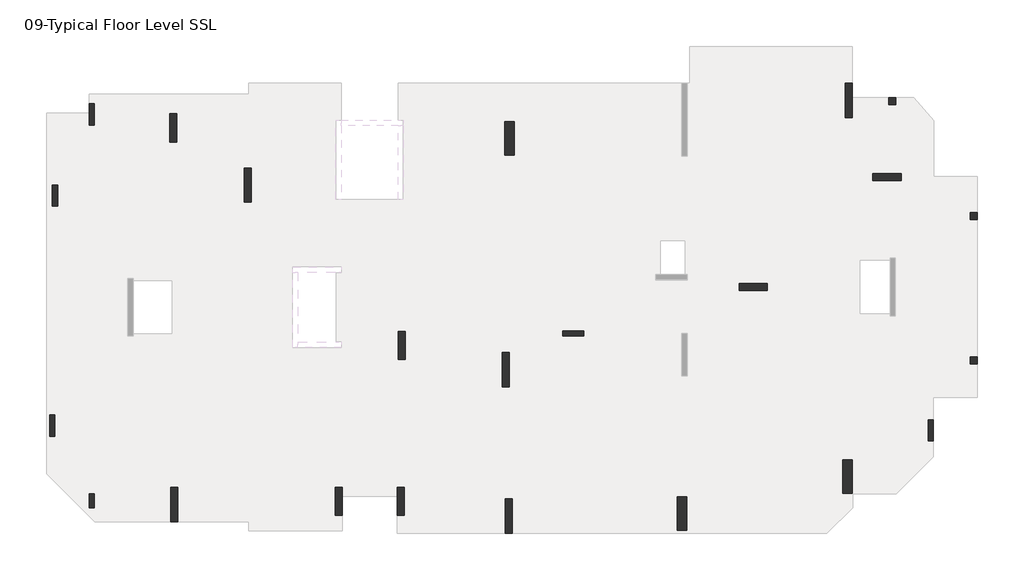
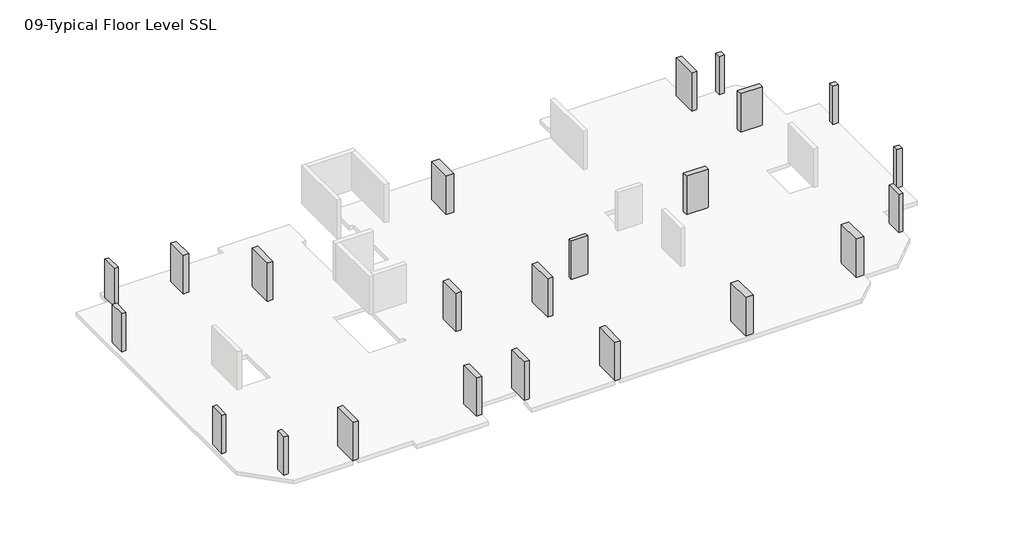
# One storey, part 2 of 2: 23 columns.
"""IFC4 building model written with IfcOpenShell, lengths in millimetres."""

import ifcopenshell
import ifcopenshell.guid

model = None  # the IFC model being written
_history = None  # IfcOwnerHistory: only IFC2X3 demands one
_inside = {}  # id of a spatial element -> (the spatial element, [elements in it])
_under = {}  # id of a project, library or spatial element -> (it, [spatial elements below it])
_declared = {}  # id of a project -> (the project, [libraries it declares])
_typed = {}  # id of a type object -> (the type object, [elements of that type])
_made_of = {}  # id of a material, layer set ... -> (it, [elements and type objects made of it])


def new_model(schema):
    """Start an empty IFC model of exactly this schema.

    Asked for "IFC4X3", IfcOpenShell would pick the latest addendum, in which some entities
    have other attributes; the version numbers below select the first issue.
    IFC2X3 requires an IfcOwnerHistory on every rooted entity: one is made here for all.
    """
    global model, _history
    if schema == "IFC4X3":
        model = ifcopenshell.file(schema_version=(4, 3, 0, 0))
    else:
        model = ifcopenshell.file(schema=schema)
    _inside.clear()
    _under.clear()
    _declared.clear()
    _typed.clear()
    _made_of.clear()
    _history = None
    if model.schema == "IFC2X3":
        org = make("IfcOrganization", Name="unknown")
        user = make(
            "IfcPersonAndOrganization",
            ThePerson=make("IfcPerson", FamilyName="unknown"),
            TheOrganization=org,
        )
        app = make(
            "IfcApplication",
            ApplicationDeveloper=org,
            Version="unknown",
            ApplicationFullName="unknown",
            ApplicationIdentifier="unknown",
        )
        _history = make(
            "IfcOwnerHistory",
            OwningUser=user,
            OwningApplication=app,
            ChangeAction="ADDED",
            CreationDate=0,
        )
    return model


def make(cls, **values):
    """One entity of the class cls with the attributes given. An attribute that is None is left unset."""
    return model.create_entity(
        cls, **{name: value for name, value in values.items() if value is not None}
    )


def rooted(cls, **values):
    """An entity with a GlobalId (a new one), such as an element, a storey or a relation."""
    return make(cls, GlobalId=ifcopenshell.guid.new(), OwnerHistory=_history, **values)


def si_unit(unit_type, name, prefix=None):
    """IfcSIUnit, for example si_unit("LENGTHUNIT", "METRE", prefix="MILLI")."""
    return make("IfcSIUnit", UnitType=unit_type, Prefix=prefix, Name=name)


def assignment(units):
    """IfcUnitAssignment: the units of a project."""
    return None if units is None else make("IfcUnitAssignment", Units=units)


def point(xyz):
    """IfcCartesianPoint."""
    return None if xyz is None else make("IfcCartesianPoint", Coordinates=xyz)


def direction(xyz):
    """IfcDirection."""
    return None if xyz is None else make("IfcDirection", DirectionRatios=xyz)


def frame(location, z_axis=None, x_axis=None):
    """IfcAxis2Placement3D, a coordinate frame: its origin and axes. An axis left out is left unset."""
    return make(
        "IfcAxis2Placement3D",
        Location=point(location),
        Axis=direction(z_axis),
        RefDirection=direction(x_axis),
    )


def origin():
    """The frame at (0, 0, 0) with its axes left unset."""
    return frame((0.0, 0.0, 0.0))


def place(relative_to, where):
    """IfcLocalPlacement: puts the frame where relative to a parent placement (None: the world)."""
    return make(
        "IfcLocalPlacement", PlacementRelTo=relative_to, RelativePlacement=where
    )


def context(
    kind, dimensions, precision=None, world=None, true_north=None, identifier=None
):
    """IfcGeometricRepresentationContext, for example the 3D "Model" context."""
    return make(
        "IfcGeometricRepresentationContext",
        ContextIdentifier=identifier,
        ContextType=kind,
        CoordinateSpaceDimension=dimensions,
        Precision=precision,
        WorldCoordinateSystem=world,
        TrueNorth=true_north,
    )


def project(units=None, contexts=None):
    """IfcProject with its units and contexts."""
    return rooted(
        "IfcProject",
        Name="project",
        RepresentationContexts=contexts,
        UnitsInContext=assignment(units),
    )


def spatial(cls, under=None, at=None, **own):
    """A site, building, storey or space (cls), placed at a placement, below another one or the project."""
    s = rooted(cls, ObjectPlacement=at, **own)
    if under is not None:
        _under.setdefault(under.id(), (under, []))[1].append(s)
    return s


def faces_of(points, faces, orient=None, outer=None):
    """IfcFace entities. A face is a list of loops; a loop is a list of indices into points, from 0.

    orient and outer hold one flag for each loop. By default every Orientation is true, the
    first loop of a face is its IfcFaceOuterBound and the others are IfcFaceBound.
    """
    made = []
    for i, loops in enumerate(faces):
        bounds = []
        for j, loop in enumerate(loops):
            is_outer = j == 0 if outer is None else outer[i][j]
            bounds.append(
                make(
                    "IfcFaceOuterBound" if is_outer else "IfcFaceBound",
                    Bound=make("IfcPolyLoop", Polygon=[points[k] for k in loop]),
                    Orientation=True if orient is None else orient[i][j],
                )
            )
        made.append(make("IfcFace", Bounds=bounds))
    return made


def faceted_brep(points, faces, orient=None, outer=None, voids=None):
    """IfcFacetedBrep: a solid bounded by flat faces; with voids (closed shells), ...WithVoids."""
    shared = [point(p) for p in points]
    hull = make("IfcClosedShell", CfsFaces=faces_of(shared, faces, orient, outer))
    if voids is None:
        return make("IfcFacetedBrep", Outer=hull)
    return make(
        "IfcFacetedBrepWithVoids",
        Outer=hull,
        Voids=[
            make(cls, CfsFaces=faces_of(shared, fs, o, b)) for cls, fs, o, b in voids
        ],
    )


def shape(context_of_items, identifier, shape_type, items):
    """IfcShapeRepresentation: the items that make up one representation, for example the "Body"."""
    return make(
        "IfcShapeRepresentation",
        ContextOfItems=context_of_items,
        RepresentationIdentifier=identifier,
        RepresentationType=shape_type,
        Items=items,
    )


def made_of(thing, what):
    """Note that an element or type object is made of a material, layer set ...; save() writes the relation."""
    if what is not None:
        _made_of.setdefault(what.id(), (what, []))[1].append(thing)
    return thing


def element(
    cls,
    number,
    at=None,
    inside=None,
    cuts=None,
    type_object=None,
    material=None,
    context=None,
    identifier="Body",
    shape_type=None,
    held_by="IfcProductDefinitionShape",
    body=None,
    shapes=None,
    **own,
):
    """One element of the class cls, such as IfcWall. Its Tag is "e" and its number.

    at: its placement. inside: the storey or other place that contains it. cuts: it is an
    opening in that element (IfcRelVoidsElement). A single representation is given by context,
    identifier, shape_type and body (its items); several are given by shapes. held_by: the class
    of the entity that holds the representations. save() writes the other relations.
    """
    e = rooted(cls, Tag="e%d" % number, ObjectPlacement=at, **own)
    if body is not None:
        shapes = [shape(context, identifier, shape_type, body)]
    if shapes is not None:
        e.Representation = make(held_by, Representations=shapes)
    if inside is not None:
        _inside.setdefault(inside.id(), (inside, []))[1].append(e)
    if cuts is not None:
        rooted(
            "IfcRelVoidsElement", RelatingBuildingElement=cuts, RelatedOpeningElement=e
        )
    if type_object is not None:
        _typed.setdefault(type_object.id(), (type_object, []))[1].append(e)
    return made_of(e, material)


def aggregate(whole, parts):
    """IfcRelAggregates: a whole, such as a stair, and the parts it consists of."""
    return rooted("IfcRelAggregates", RelatingObject=whole, RelatedObjects=parts)


def save(model, path):
    """Write the relations noted so far, then the file.

    IfcRelAggregates (storeys below a building ...), IfcRelContainedInSpatialStructure (elements
    in a storey), IfcRelDefinesByType, IfcRelAssociatesMaterial and IfcRelDeclares: one each for
    every whole, place, type object, material and project.
    """
    for whole, parts in _under.values():
        aggregate(whole, parts)
    for where, things in _inside.values():
        rooted(
            "IfcRelContainedInSpatialStructure",
            RelatedElements=things,
            RelatingStructure=where,
        )
    for kind, things in _typed.values():
        rooted("IfcRelDefinesByType", RelatedObjects=things, RelatingType=kind)
    for what, things in _made_of.values():
        rooted("IfcRelAssociatesMaterial", RelatedObjects=things, RelatingMaterial=what)
    for by, libraries in _declared.values():
        rooted("IfcRelDeclares", RelatingContext=by, RelatedDefinitions=libraries)
    model.write(path)


model = new_model("IFC4")

# Units and contexts
model_context = context("Model", 3, world=origin())
ifc_project = project(units=[si_unit("LENGTHUNIT", "METRE", prefix="MILLI")], contexts=[model_context])

# Site, building, storey
site = spatial("IfcSite", under=ifc_project)
building = spatial("IfcBuilding", under=site)
storey = spatial("IfcBuildingStorey", under=building, Name="09-Typical Floor Level SSL", Elevation=21000.0)

# Columns
placement = place(None, origin())
element("IfcColumn", 1, ObjectType="M_Concrete-Rectangular-Column : C-1 (400 x 400mm)", at=placement, inside=storey, context=model_context, shape_type="Brep", body=[
    faceted_brep([(52549.9999998, 16712.0, 21000.0), (52549.9999998, 16312.0, 21000.0), (52149.9999998, 16312.0, 21000.0), (52149.9999998, 16712.0, 21000.0), (52549.9999998, 16712.0, 24000.0), (52549.9999998, 16312.0, 24000.0), (52549.9999998, 16312.0, 23700.0), (52549.9999998, 16712.0, 23700.0), (52149.9999998, 16312.0, 24000.0), (52149.9999998, 16312.0, 23700.0), (52149.9999998, 16712.0, 24000.0), (52149.9999998, 16712.0, 23700.0)], [[[0, 1, 2, 3]], [[4, 5, 6, 1, 0, 7]], [[5, 8, 9, 2, 1, 6]], [[8, 10, 11, 3, 2, 9]], [[10, 4, 7, 0, 3, 11]], [[4, 10, 8, 5]]]),
])
element("IfcColumn", 2, ObjectType="M_Concrete-Rectangular-Column : C-1 (400 x 400mm)", at=placement, inside=storey, context=model_context, shape_type="Brep", body=[
    faceted_brep([(47898.6337868, 23252.0, 21000.0), (47898.6337868, 22852.0, 21000.0), (47498.6337868, 22852.0, 21000.0), (47498.6337868, 23252.0, 21000.0), (47898.6337868, 23252.0, 24000.0), (47898.6337868, 22852.0, 24000.0), (47898.6337868, 22852.0, 23700.0), (47498.6337868, 22852.0, 24000.0), (47498.6337868, 22852.0, 23700.0), (47498.6337868, 23252.0, 24000.0)], [[[0, 1, 2, 3]], [[4, 5, 6, 1, 0]], [[5, 7, 8, 2, 1, 6]], [[7, 9, 3, 2, 8]], [[9, 4, 0, 3]], [[4, 9, 7, 5]]]),
])
element("IfcColumn", 3, ObjectType="M_Concrete-Rectangular-Column : C-1 (400 x 400mm)", at=placement, inside=storey, context=model_context, shape_type="Brep", body=[
    faceted_brep([(52549.9999998, 8504.0039609, 21000.0), (52549.9999998, 8104.0039609, 21000.0), (52149.9999998, 8104.0039609, 21000.0), (52149.9999998, 8504.0039609, 21000.0), (52549.9999998, 8504.0039609, 24000.0), (52549.9999998, 8104.0039609, 24000.0), (52549.9999998, 8104.0039609, 23700.0), (52549.9999998, 8504.0039609, 23700.0), (52149.9999998, 8104.0039609, 24000.0), (52149.9999998, 8104.0039609, 23700.0), (52149.9999998, 8504.0039609, 24000.0), (52149.9999998, 8504.0039609, 23700.0)], [[[0, 1, 2, 3]], [[4, 5, 6, 1, 0, 7]], [[5, 8, 9, 2, 1, 6]], [[8, 10, 11, 3, 2, 9]], [[10, 4, 7, 0, 3, 11]], [[4, 10, 8, 5]]]),
])
element("IfcColumn", 4, ObjectType="M_Concrete-Rectangular-Column : C-2 (300 x 800mm)", at=placement, inside=storey, context=model_context, shape_type="Brep", body=[
    faceted_brep([(2352.0, 728.0, 21000.0), (2352.0, -72.0, 21000.0), (2052.0, -72.0, 21000.0), (2052.0, 728.0, 21000.0), (2352.0, 728.0, 24000.0), (2352.0, -72.0, 24000.0), (2352.0, -72.0, 23700.0), (2352.0, 728.0, 23700.0), (2052.0, -72.0, 24000.0), (2052.0, -72.0, 23700.0), (2052.0, 728.0, 24000.0), (2052.0, 728.0, 23700.0)], [[[0, 1, 2, 3]], [[4, 5, 6, 1, 0, 7]], [[5, 8, 9, 2, 1, 6]], [[8, 10, 11, 3, 2, 9]], [[10, 4, 7, 0, 3, 11]], [[4, 10, 8, 5]]]),
])
element("IfcColumn", 5, ObjectType="M_Concrete-Rectangular-Column : C-3(300 x 1200mm)", at=placement, inside=storey, context=model_context, shape_type="Brep", body=[
    faceted_brep([(2352.0, 22908.0000656, 21000.0), (2352.0, 21708.0000656, 21000.0), (2052.0, 21708.0000656, 21000.0), (2052.0, 22908.0000656, 21000.0), (2352.0, 22908.0000656, 24000.0), (2352.0, 21708.0000656, 24000.0), (2352.0, 21708.0000656, 23700.0), (2352.0, 22908.0000656, 23700.0), (2052.0, 21708.0000656, 24000.0), (2052.0, 21708.0000656, 23700.0), (2052.0, 22380.0004589, 24000.0), (2052.0, 22908.0000656, 24000.0), (2052.0, 22908.0000656, 23700.0)], [[[0, 1, 2, 3]], [[4, 5, 6, 1, 0, 7]], [[5, 8, 9, 2, 1, 6]], [[8, 10, 11, 12, 3, 2, 9]], [[11, 4, 7, 0, 3, 12]], [[4, 11, 10, 8, 5]]]),
])
element("IfcColumn", 6, ObjectType="M_Concrete-Rectangular-Column : C-3(300 x 1200mm)", at=placement, inside=storey, context=model_context, shape_type="Brep", body=[
    faceted_brep([(257.9999999, 18288.0, 21000.0), (257.9999999, 17088.0, 21000.0), (-42.0000001, 17088.0, 21000.0), (-42.0000001, 18288.0, 21000.0), (257.9999999, 18288.0, 24000.0), (257.9999999, 17088.0, 24000.0), (257.9999999, 17088.0, 23700.0), (257.9999999, 18288.0, 23700.0), (-42.0000001, 17088.0, 24000.0), (-42.0000001, 17088.0, 23700.0), (-42.0000001, 18288.0, 24000.0), (-42.0000001, 18288.0, 23700.0)], [[[0, 1, 2, 3]], [[4, 5, 6, 1, 0, 7]], [[5, 8, 9, 2, 1, 6]], [[8, 10, 11, 3, 2, 9]], [[10, 4, 7, 0, 3, 11]], [[4, 10, 8, 5]]]),
])
element("IfcColumn", 7, ObjectType="M_Concrete-Rectangular-Column : C-3(300 x 1200mm)", at=placement, inside=storey, context=model_context, shape_type="Brep", body=[
    faceted_brep([(108.001803, 5201.9999858, 21000.0), (108.001803, 4001.9999858, 21000.0), (-191.998197, 4001.9999858, 21000.0), (-191.998197, 5201.9999858, 21000.0), (108.001803, 5201.9999858, 24000.0), (108.001803, 4001.9999858, 24000.0), (108.001803, 4001.9999858, 23700.0), (108.001803, 5201.9999858, 23700.0), (-191.998197, 4001.9999858, 24000.0), (-191.998197, 4001.9999858, 23700.0), (-191.998197, 5201.9999858, 24000.0), (-191.998197, 5201.9999858, 23700.0)], [[[0, 1, 2, 3]], [[4, 5, 6, 1, 0, 7]], [[5, 8, 9, 2, 1, 6]], [[8, 10, 11, 3, 2, 9]], [[10, 4, 7, 0, 3, 11]], [[4, 10, 8, 5]]]),
])
element("IfcColumn", 8, ObjectType="M_Concrete-Rectangular-Column : C-3(300 x 1200mm)", at=placement, inside=storey, context=model_context, shape_type="Brep", body=[
    faceted_brep([(50046.0009271, 4931.9999929, 21000.0), (50046.0009271, 3731.9999929, 21000.0), (49746.0009271, 3731.9999929, 21000.0), (49746.0009271, 4931.9999929, 21000.0), (50046.0009271, 4931.9999929, 24000.0), (50046.0009271, 3731.9999929, 24000.0), (50046.0009271, 3731.9999929, 23700.0), (50046.0009271, 4931.9999929, 23700.0), (49746.0009271, 3731.9999929, 24000.0), (49746.0009271, 3731.9999929, 23700.0), (49746.0009271, 4931.9999929, 24000.0), (49746.0009271, 4931.9999929, 23700.0)], [[[0, 1, 2, 3]], [[4, 5, 6, 1, 0, 7]], [[5, 8, 9, 2, 1, 6]], [[8, 10, 11, 3, 2, 9]], [[10, 4, 7, 0, 3, 11]], [[4, 10, 8, 5]]]),
])
element("IfcColumn", 9, ObjectType="M_Concrete-Rectangular-Column : C-3(300 x 1200mm)", at=placement, inside=storey, context=model_context, shape_type="Brep", body=[
    faceted_brep([(28975.9999998, 9996.0000019, 21000.0), (30175.9999998, 9996.0000019, 21000.0), (30175.9999998, 9696.0000019, 21000.0), (28975.9999998, 9696.0000019, 21000.0), (28975.9999998, 9996.0000019, 24000.0), (30175.9999998, 9996.0000019, 24000.0), (30175.9999998, 9996.0000019, 23700.0), (28975.9999998, 9996.0000019, 23700.0), (30175.9999998, 9696.0000019, 24000.0), (30175.9999998, 9696.0000019, 23700.0), (28975.9999998, 9696.0000019, 24000.0), (28975.9999998, 9696.0000019, 23700.0)], [[[0, 1, 2, 3]], [[4, 5, 6, 1, 0, 7]], [[5, 8, 9, 2, 1, 6]], [[8, 10, 11, 3, 2, 9]], [[10, 4, 7, 0, 3, 11]], [[4, 10, 8, 5]]]),
])
element("IfcColumn", 10, ObjectType="M_Concrete-Rectangular-Column : C-4 (400 x 1600mm)", at=placement, inside=storey, context=model_context, shape_type="Brep", body=[
    faceted_brep([(7021.9999999, 22340.0000078, 21000.0), (7021.9999999, 20740.0000078, 21000.0), (6621.9999999, 20740.0000078, 21000.0), (6621.9999999, 22340.0000078, 21000.0), (7021.9999999, 22340.0000078, 24000.0), (7021.9999999, 20740.0000078, 24000.0), (7021.9999999, 20740.0000078, 23700.0), (7021.9999999, 22340.0000078, 23700.0), (6621.9999999, 20740.0000078, 24000.0), (6621.9999999, 20740.0000078, 23700.0), (6621.9999999, 22340.0000078, 24000.0), (6621.9999999, 22340.0000078, 23700.0)], [[[0, 1, 2, 3]], [[4, 5, 6, 1, 0, 7]], [[5, 8, 9, 2, 1, 6]], [[8, 10, 11, 3, 2, 9]], [[10, 4, 7, 0, 3, 11]], [[4, 10, 8, 5]]]),
])
element("IfcColumn", 11, ObjectType="M_Concrete-Rectangular-Column : C-4 (400 x 1600mm)", at=placement, inside=storey, context=model_context, shape_type="Brep", body=[
    faceted_brep([(19969.9997488, 1087.9955348, 21000.0), (19969.9997488, -512.0044652, 21000.0), (19569.9997488, -512.0044652, 21000.0), (19569.9997488, 1087.9955348, 21000.0), (19969.9997488, 1087.9955348, 24000.0), (19969.9997488, -512.0044652, 24000.0), (19969.9997488, -512.0044652, 23700.0), (19969.9997488, 1087.9955348, 23700.0), (19569.9997488, -512.0044652, 24000.0), (19569.9997488, -512.0044652, 23700.0), (19569.9997488, 564.000519, 24000.0), (19569.9997488, 1087.9955348, 24000.0), (19569.9997488, 1087.9955348, 23700.0)], [[[0, 1, 2, 3]], [[4, 5, 6, 1, 0, 7]], [[5, 8, 9, 2, 1, 6]], [[8, 10, 11, 12, 3, 2, 9]], [[11, 4, 7, 0, 3, 12]], [[4, 11, 10, 8, 5]]]),
])
element("IfcColumn", 12, ObjectType="M_Concrete-Rectangular-Column : C-4 (400 x 1600mm)", at=placement, inside=storey, context=model_context, shape_type="Brep", body=[
    faceted_brep([(46605.9993605, 18950.0, 21000.0), (48205.9993605, 18950.0, 21000.0), (48205.9993605, 18550.0, 21000.0), (46605.9993605, 18550.0, 21000.0), (46605.9993605, 18950.0, 24000.0), (48205.9993605, 18950.0, 24000.0), (48205.9993605, 18950.0, 23700.0), (46605.9993605, 18950.0, 23700.0), (48205.9993605, 18550.0, 24000.0), (48205.9993605, 18550.0, 23700.0), (46605.9993605, 18550.0, 24000.0), (46605.9993605, 18550.0, 23700.0)], [[[0, 1, 2, 3]], [[4, 5, 6, 1, 0, 7]], [[5, 8, 9, 2, 1, 6]], [[8, 10, 11, 3, 2, 9]], [[10, 4, 7, 0, 3, 11]], [[4, 10, 8, 5]]]),
])
element("IfcColumn", 13, ObjectType="M_Concrete-Rectangular-Column : C-5 (400 x 1600mm)", at=placement, inside=storey, context=model_context, shape_type="Brep", body=[
    faceted_brep([(20030.000009, 9955.9999979, 21000.0), (20030.000009, 8355.9999979, 21000.0), (19630.000009, 8355.9999979, 21000.0), (19630.000009, 9955.9999979, 21000.0), (20030.000009, 9955.9999979, 24000.0), (20030.000009, 8355.9999979, 24000.0), (20030.000009, 8355.9999979, 23700.0), (20030.000009, 9955.9999979, 23700.0), (19630.000009, 8355.9999979, 24000.0), (19630.000009, 8355.9999979, 23700.0), (19630.000009, 9955.9999979, 24000.0), (19630.000009, 9955.9999979, 23700.0)], [[[0, 1, 2, 3]], [[4, 5, 6, 1, 0, 7]], [[5, 8, 9, 2, 1, 6]], [[8, 10, 11, 3, 2, 9]], [[10, 4, 7, 0, 3, 11]], [[4, 10, 8, 5]]]),
])
element("IfcColumn", 14, ObjectType="M_Concrete-Rectangular-Column : C-5 (400 x 1600mm)", at=placement, inside=storey, context=model_context, shape_type="Brep", body=[
    faceted_brep([(16429.9999981, 1088.0, 21000.0), (16429.9999981, -512.0, 21000.0), (16029.9999981, -512.0, 21000.0), (16029.9999981, 1088.0, 21000.0), (16429.9999981, 1088.0, 24000.0), (16429.9999981, 564.000519, 24000.0), (16429.9999981, -512.0, 24000.0), (16429.9999981, -512.0, 23700.0), (16429.9999981, 1088.0, 23700.0), (16029.9999981, -512.0, 24000.0), (16029.9999981, -512.0, 23700.0), (16029.9999981, 1088.0, 24000.0), (16029.9999981, 1088.0, 23700.0)], [[[0, 1, 2, 3]], [[4, 5, 6, 7, 1, 0, 8]], [[6, 9, 10, 2, 1, 7]], [[9, 11, 12, 3, 2, 10]], [[11, 4, 8, 0, 3, 12]], [[4, 11, 9, 6, 5]]]),
])
element("IfcColumn", 15, ObjectType="M_Concrete-Rectangular-Column : C-5 (400 x 1600mm)", at=placement, inside=storey, context=model_context, shape_type="Brep", body=[
    faceted_brep([(38998.0014887, 12692.0079212, 21000.0), (40598.0014887, 12692.0079212, 21000.0), (40598.0014887, 12292.0079212, 21000.0), (38998.0014887, 12292.0079212, 21000.0), (38998.0014887, 12692.0079212, 24000.0), (40598.0014887, 12692.0079212, 24000.0), (40598.0014887, 12692.0079212, 23700.0), (38998.0014887, 12692.0079212, 23700.0), (40598.0014887, 12292.0079212, 24000.0), (40598.0014887, 12292.0079212, 23700.0), (38998.0014887, 12292.0079212, 24000.0), (38998.0014887, 12292.0079212, 23700.0)], [[[0, 1, 2, 3]], [[4, 5, 6, 1, 0, 7]], [[5, 8, 9, 2, 1, 6]], [[8, 10, 11, 3, 2, 9]], [[10, 4, 7, 0, 3, 11]], [[4, 10, 8, 5]]]),
])
element("IfcColumn", 16, ObjectType="M_Concrete-Rectangular-Column : C-6 (400 x 1950mm)", at=placement, inside=storey, context=model_context, shape_type="Brep", body=[
    faceted_brep([(11270.0000427, 19262.9999996, 21000.0), (11270.0000427, 17312.9999996, 21000.0), (10870.0000427, 17312.9999996, 21000.0), (10870.0000427, 19262.9999996, 21000.0), (11270.0000427, 19262.9999996, 24000.0), (11270.0000427, 17312.9999996, 24000.0), (11270.0000427, 17312.9999996, 23700.0), (11270.0000427, 19262.9999996, 23700.0), (10870.0000427, 17312.9999996, 24000.0), (10870.0000427, 17312.9999996, 23700.0), (10870.0000427, 19262.9999996, 24000.0), (10870.0000427, 19262.9999996, 23700.0)], [[[0, 1, 2, 3]], [[4, 5, 6, 1, 0, 7]], [[5, 8, 9, 2, 1, 6]], [[8, 10, 11, 3, 2, 9]], [[10, 4, 7, 0, 3, 11]], [[4, 10, 8, 5]]]),
])
element("IfcColumn", 17, ObjectType="M_Concrete-Rectangular-Column : C-6 (400 x 1950mm)", at=placement, inside=storey, context=model_context, shape_type="Brep", body=[
    faceted_brep([(7082.0000416, 1083.0000153, 21000.0), (7082.0000416, -866.9999847, 21000.0), (6682.0000416, -866.9999847, 21000.0), (6682.0000416, 1083.0000153, 21000.0), (7082.0000416, 1083.0000153, 24000.0), (7082.0000416, -866.9999847, 24000.0), (7082.0000416, -866.9999847, 23700.0), (7082.0000416, 1083.0000153, 23700.0), (6682.0000416, -866.9999847, 24000.0), (6682.0000416, -866.9999847, 23700.0), (6682.0000416, 1083.0000153, 24000.0), (6682.0000416, 1083.0000153, 23700.0)], [[[0, 1, 2, 3]], [[4, 5, 6, 1, 0, 7]], [[5, 8, 9, 2, 1, 6]], [[8, 10, 11, 3, 2, 9]], [[10, 4, 7, 0, 3, 11]], [[4, 10, 8, 5]]]),
])
element("IfcColumn", 18, ObjectType="M_Concrete-Rectangular-Column : C-6 (400 x 1950mm)", at=placement, inside=storey, context=model_context, shape_type="Brep", body=[
    faceted_brep([(26113.9999998, 422.995535, 21000.0), (26113.9999998, -1527.004465, 21000.0), (25713.9999998, -1527.004465, 21000.0), (25713.9999998, 422.995535, 21000.0), (26113.9999998, 422.995535, 24000.0), (26113.9999998, -1527.004465, 24000.0), (26113.9999998, -1527.004465, 23700.0), (26113.9999998, 422.995535, 23700.0), (25713.9999998, -1527.004465, 24000.0), (25713.9999998, -1527.004465, 23700.0), (25713.9999998, 422.995535, 24000.0), (25713.9999998, 422.995535, 23700.0)], [[[0, 1, 2, 3]], [[4, 5, 6, 1, 0, 7]], [[5, 8, 9, 2, 1, 6]], [[8, 10, 11, 3, 2, 9]], [[10, 4, 7, 0, 3, 11]], [[4, 10, 8, 5]]]),
])
element("IfcColumn", 19, ObjectType="M_Concrete-Rectangular-Column : C-6 (400 x 1950mm)", at=placement, inside=storey, context=model_context, shape_type="Brep", body=[
    faceted_brep([(45446.0007483, 24087.0, 21000.0), (45446.0007483, 22137.0, 21000.0), (45046.0007483, 22137.0, 21000.0), (45046.0007483, 24087.0, 21000.0), (45446.0007483, 24087.0, 24000.0), (45446.0007483, 23252.0000315, 24000.0), (45446.0007483, 22137.0, 24000.0), (45446.0007483, 22137.0, 23700.0), (45446.0007483, 24087.0, 23700.0), (45046.0007483, 22137.0, 24000.0), (45046.0007483, 22137.0, 23700.0), (45046.0007483, 24087.0, 24000.0), (45046.0007483, 24087.0, 23700.0)], [[[0, 1, 2, 3]], [[4, 5, 6, 7, 1, 0, 8]], [[6, 9, 10, 2, 1, 7]], [[9, 11, 12, 3, 2, 10]], [[11, 4, 8, 0, 3, 12]], [[4, 11, 9, 6, 5]]]),
])
element("IfcColumn", 20, ObjectType="M_Concrete-Rectangular-Column : C-6 (400 x 1950mm)", at=placement, inside=storey, context=model_context, shape_type="Brep", body=[
    faceted_brep([(25934.0000455, 8751.0001824, 21000.0), (25934.0000455, 6801.0001824, 21000.0), (25534.0000455, 6801.0001824, 21000.0), (25534.0000455, 8751.0001824, 21000.0), (25934.0000455, 8751.0001824, 24000.0), (25934.0000455, 6801.0001824, 24000.0), (25934.0000455, 6801.0001824, 23700.0), (25934.0000455, 8751.0001824, 23700.0), (25534.0000455, 6801.0001824, 24000.0), (25534.0000455, 6801.0001824, 23700.0), (25534.0000455, 8751.0001824, 24000.0), (25534.0000455, 8751.0001824, 23700.0)], [[[0, 1, 2, 3]], [[4, 5, 6, 1, 0, 7]], [[5, 8, 9, 2, 1, 6]], [[8, 10, 11, 3, 2, 9]], [[10, 4, 7, 0, 3, 11]], [[4, 10, 8, 5]]]),
])
element("IfcColumn", 21, ObjectType="M_Concrete-Rectangular-Column : C-7 (550 x 1900mm)", at=placement, inside=storey, context=model_context, shape_type="Brep", body=[
    faceted_brep([(36035.9999998, 548.0007983, 21000.0), (36035.9999998, -1351.9992017, 21000.0), (35485.9999998, -1351.9992017, 21000.0), (35485.9999998, 548.0007983, 21000.0), (36035.9999998, 548.0007983, 24000.0), (36035.9999998, -1351.9992017, 24000.0), (36035.9999998, -1351.9992017, 23700.0), (36035.9999998, 548.0007983, 23700.0), (35485.9999998, -1351.9992017, 24000.0), (35485.9999998, -1351.9992017, 23700.0), (35485.9999998, 548.0007983, 24000.0), (35485.9999998, 548.0007983, 23700.0)], [[[0, 1, 2, 3]], [[4, 5, 6, 1, 0, 7]], [[5, 8, 9, 2, 1, 6]], [[8, 10, 11, 3, 2, 9]], [[10, 4, 7, 0, 3, 11]], [[4, 10, 8, 5]]]),
])
element("IfcColumn", 22, ObjectType="M_Concrete-Rectangular-Column : C-7 (550 x 1900mm)", at=placement, inside=storey, context=model_context, shape_type="Brep", body=[
    faceted_brep([(45443.9999998, 2648.0, 21000.0), (45443.9999998, 748.0, 21000.0), (44893.9999998, 748.0, 21000.0), (44893.9999998, 2648.0, 21000.0), (45443.9999998, 2648.0, 24000.0), (45443.9999998, 748.0, 24000.0), (45443.9999998, 748.0, 23700.0), (45443.9999998, 2648.0, 23700.0), (44893.9999998, 748.0, 24000.0), (44893.9999998, 748.0, 23700.0), (44893.9999998, 2648.0, 24000.0), (44893.9999998, 2648.0, 23700.0)], [[[0, 1, 2, 3]], [[4, 5, 6, 1, 0, 7]], [[5, 8, 9, 2, 1, 6]], [[8, 10, 11, 3, 2, 9]], [[10, 4, 7, 0, 3, 11]], [[4, 10, 8, 5]]]),
])
element("IfcColumn", 23, ObjectType="M_Concrete-Rectangular-Column : C-7 (550 x 1900mm)", at=placement, inside=storey, context=model_context, shape_type="Brep", body=[
    faceted_brep([(26218.9999998, 21900.0, 21000.0), (26218.9999998, 20000.0, 21000.0), (25668.9999998, 20000.0, 21000.0), (25668.9999998, 21900.0, 21000.0), (26218.9999998, 21900.0, 24000.0), (26218.9999998, 20000.0, 24000.0), (26218.9999998, 20000.0, 23700.0), (26218.9999998, 21900.0, 23700.0), (25668.9999998, 20000.0, 24000.0), (25668.9999998, 20000.0, 23700.0), (25668.9999998, 21900.0, 24000.0), (25668.9999998, 21900.0, 23700.0)], [[[0, 1, 2, 3]], [[4, 5, 6, 1, 0, 7]], [[5, 8, 9, 2, 1, 6]], [[8, 10, 11, 3, 2, 9]], [[10, 4, 7, 0, 3, 11]], [[4, 10, 8, 5]]]),
])

save(model, "model.ifc")

# Revit data of these elements
# Type "M_Concrete-Rectangular-Column : C-1 (400 x 400mm)"
#   Type Mark = "C01"
#   b = 400 mm
#   h = 400 mm
#   Structural Material [instance default] = Concrete, Cast-in-Place gray
# Type "M_Concrete-Rectangular-Column : C-2 (300 x 800mm)"
#   Type Mark = "C02"
#   b = 300 mm
#   h = 800 mm
#   Structural Material [instance default] = Concrete, Cast-in-Place gray
# Type "M_Concrete-Rectangular-Column : C-3(300 x 1200mm)"
#   Type Mark = "C03"
#   b = 300 mm
#   h = 1200 mm
#   Structural Material [instance default] = Concrete, Cast-in-Place gray
# Type "M_Concrete-Rectangular-Column : C-4 (400 x 1600mm)"
#   Type Mark = "C04"
#   b = 400 mm
#   h = 1600 mm
#   Structural Material [instance default] = Concrete, Cast-in-Place gray
# Type "M_Concrete-Rectangular-Column : C-5 (400 x 1600mm)"
#   Type Mark = "C05"
#   b = 400 mm
#   h = 1600 mm
#   Structural Material [instance default] = Concrete, Cast-in-Place gray
# Type "M_Concrete-Rectangular-Column : C-6 (400 x 1950mm)"
#   Type Mark = "C06"
#   b = 400 mm
#   h = 1950 mm
#   Structural Material [instance default] = Concrete, Cast-in-Place gray
# Type "M_Concrete-Rectangular-Column : C-7 (550 x 1900mm)"
#   Type Mark = "C07"
#   b = 550 mm
#   h = 1900 mm
#   Structural Material [instance default] = Concrete, Cast-in-Place gray
# Elements 1, 2, 3 (IfcColumn, "M_Concrete-Rectangular-Column : C-1 (400 x 400mm)")
#   Structural Material = Concrete-RC
#   Phase Created = New Construction
#   Materials on its faces: "Concrete-RC"
# Element 4 (IfcColumn, "M_Concrete-Rectangular-Column : C-2 (300 x 800mm)")
#   Structural Material = Concrete-RC
#   Phase Created = New Construction
#   Materials on its faces: "Concrete-RC"
# Elements 5, 6, 7, 8, 9 (IfcColumn, "M_Concrete-Rectangular-Column : C-3(300 x 1200mm)")
#   Structural Material = Concrete-RC
#   Phase Created = New Construction
#   Materials on its faces: "Concrete-RC"
# Elements 10, 11, 12 (IfcColumn, "M_Concrete-Rectangular-Column : C-4 (400 x 1600mm)")
#   Structural Material = Concrete-RC
#   Phase Created = New Construction
#   Materials on its faces: "Concrete-RC"
# Elements 13, 14, 15 (IfcColumn, "M_Concrete-Rectangular-Column : C-5 (400 x 1600mm)")
#   Structural Material = Concrete-RC
#   Phase Created = New Construction
#   Materials on its faces: "Concrete-RC"
# Elements 16, 17, 18, 19, 20 (IfcColumn, "M_Concrete-Rectangular-Column : C-6 (400 x 1950mm)")
#   Structural Material = Concrete-RC
#   Phase Created = New Construction
#   Materials on its faces: "Concrete-RC"
# Elements 21, 22, 23 (IfcColumn, "M_Concrete-Rectangular-Column : C-7 (550 x 1900mm)")
#   Structural Material = Concrete-RC
#   Phase Created = New Construction
#   Materials on its faces: "Concrete-RC"
# Materials
#   "Concrete, Cast-in-Place gray": class "Concrete", colour RGB 192 192 192, transparency 0, Description = "Cast-in-place concrete", Cost = 0
#   "Concrete-RC": class "Concrete", colour RGB 128 128 128, transparency 0, Description = "High strength concrete", Cost = 0
